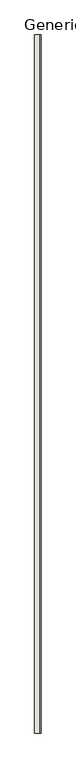
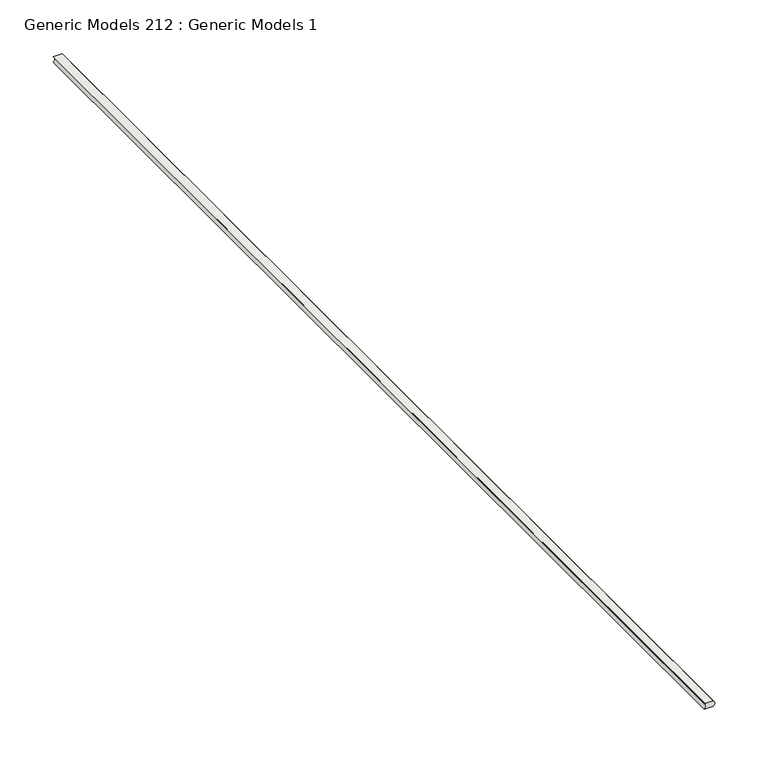
"""IFC4 building model written with IfcOpenShell, lengths in millimetres: wall geometry, Generic Models 212 : Generic Models 1."""

from ifc_helpers import new_model, si_unit, point, frame, frame_2d, origin, place, context, project, spatial, polyline, circle_curve, trimmed, segment, composite_curve, outline, extrude, source, transform, mapped, element, save


def generic_models_212_generic_models_1_7e6a8deb(model_context):
    return source(origin(), model_context, "Body", "SweptSolid", [
        extrude(outline(composite_curve([segment(polyline([(3048.0, 49758.6), (3048.0, 49768.125)]), True, "CONTINUOUS"), segment(trimmed(circle_curve(frame_2d((3051.175, 49765.2102595)), 4.3100275), [point((3048.0, 49768.125))], [point((3054.35, 49768.125))], False, "CARTESIAN"), True, "CONTINUOUS"), segment(polyline([(3054.35, 49768.125), (3054.35, 49758.6)]), True, "CONTINUOUS"), segment(trimmed(circle_curve(frame_2d((3051.175, 49755.6852595)), 4.3100275), [point((3054.35, 49758.6))], [point((3048.0, 49758.6))], True, "CARTESIAN"), True, "CONTINUOUS")], self_intersect=False)), frame((0.0, 0.0, 0.0), z_axis=(0.0, 1.0, 0.0), x_axis=(0.0, 0.0, 1.0)), (0.0, 0.0, 1.0), 1219.2),
    ])


if __name__ == "__main__":
    model = new_model("IFC4")
    model_context = context("Model", 3, world=origin())
    ifc_project = project(units=[si_unit("LENGTHUNIT", "METRE", prefix="MILLI")], contexts=[model_context])
    site = spatial("IfcSite", under=ifc_project)
    building = spatial("IfcBuilding", under=site)
    placement = place(None, origin())
    generic_models_212_generic_models_1_shape = generic_models_212_generic_models_1_7e6a8deb(model_context)
    element("IfcWall", 1, ObjectType="Generic Models 212 : Generic Models 1", at=placement, inside=building, context=model_context, shape_type="MappedRepresentation", body=[
        mapped(generic_models_212_generic_models_1_shape, transform((0.0, 0.0, 0.0), x_axis=(1.0, 0.0, 0.0), y_axis=(0.0, 1.0, 0.0), z_axis=(0.0, 0.0, 1.0))),
    ])
    save(model, "model.ifc")

# Revit data of these elements
# Element 1 (IfcWall, "Generic Models 212 : Generic Models 1")
#   Materials on its faces: "ACOUSTICAL SEALANT"
# Materials
#   "ACOUSTICAL SEALANT": class "Unassigned", colour RGB 120 120 120, transparency 0, Cost = 0
